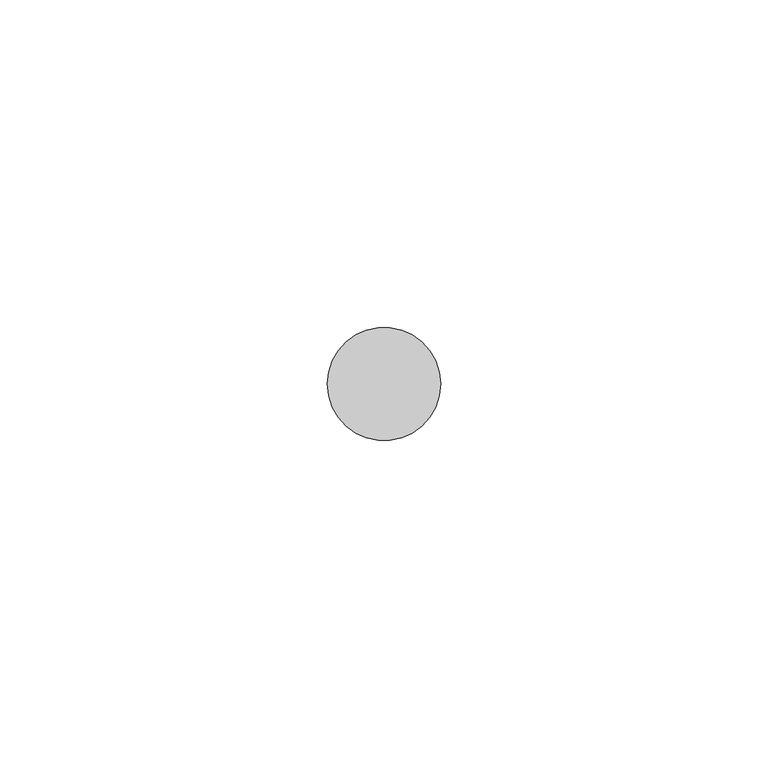
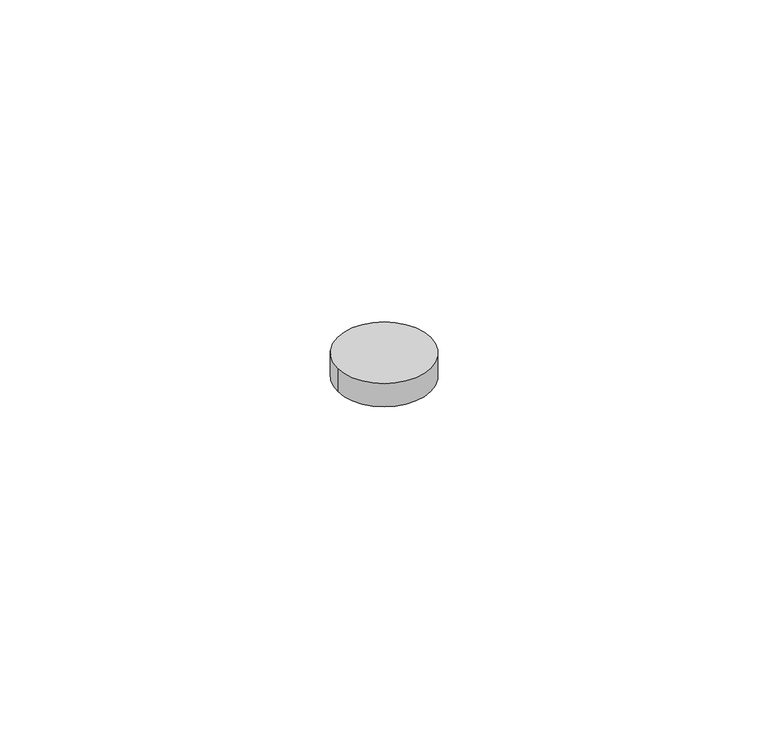
"""IFC4 building model written with IfcOpenShell, lengths in millimetres: proxy geometry, Hinge Pin Keeper17 : Hinge Pin Keeper."""

import ifcopenshell
import ifcopenshell.guid

model = None  # the IFC model being written
_history = None  # IfcOwnerHistory: only IFC2X3 demands one
_inside = {}  # id of a spatial element -> (the spatial element, [elements in it])
_under = {}  # id of a project, library or spatial element -> (it, [spatial elements below it])
_declared = {}  # id of a project -> (the project, [libraries it declares])
_typed = {}  # id of a type object -> (the type object, [elements of that type])
_made_of = {}  # id of a material, layer set ... -> (it, [elements and type objects made of it])


def new_model(schema):
    """Start an empty IFC model of exactly this schema.

    Asked for "IFC4X3", IfcOpenShell would pick the latest addendum, in which some entities
    have other attributes; the version numbers below select the first issue.
    IFC2X3 requires an IfcOwnerHistory on every rooted entity: one is made here for all.
    """
    global model, _history
    if schema == "IFC4X3":
        model = ifcopenshell.file(schema_version=(4, 3, 0, 0))
    else:
        model = ifcopenshell.file(schema=schema)
    _inside.clear()
    _under.clear()
    _declared.clear()
    _typed.clear()
    _made_of.clear()
    _history = None
    if model.schema == "IFC2X3":
        org = make("IfcOrganization", Name="unknown")
        user = make(
            "IfcPersonAndOrganization",
            ThePerson=make("IfcPerson", FamilyName="unknown"),
            TheOrganization=org,
        )
        app = make(
            "IfcApplication",
            ApplicationDeveloper=org,
            Version="unknown",
            ApplicationFullName="unknown",
            ApplicationIdentifier="unknown",
        )
        _history = make(
            "IfcOwnerHistory",
            OwningUser=user,
            OwningApplication=app,
            ChangeAction="ADDED",
            CreationDate=0,
        )
    return model


def make(cls, **values):
    """One entity of the class cls with the attributes given. An attribute that is None is left unset."""
    return model.create_entity(
        cls, **{name: value for name, value in values.items() if value is not None}
    )


def rooted(cls, **values):
    """An entity with a GlobalId (a new one), such as an element, a storey or a relation."""
    return make(cls, GlobalId=ifcopenshell.guid.new(), OwnerHistory=_history, **values)


def si_unit(unit_type, name, prefix=None):
    """IfcSIUnit, for example si_unit("LENGTHUNIT", "METRE", prefix="MILLI")."""
    return make("IfcSIUnit", UnitType=unit_type, Prefix=prefix, Name=name)


def assignment(units):
    """IfcUnitAssignment: the units of a project."""
    return None if units is None else make("IfcUnitAssignment", Units=units)


def point(xyz):
    """IfcCartesianPoint."""
    return None if xyz is None else make("IfcCartesianPoint", Coordinates=xyz)


def direction(xyz):
    """IfcDirection."""
    return None if xyz is None else make("IfcDirection", DirectionRatios=xyz)


def frame(location, z_axis=None, x_axis=None):
    """IfcAxis2Placement3D, a coordinate frame: its origin and axes. An axis left out is left unset."""
    return make(
        "IfcAxis2Placement3D",
        Location=point(location),
        Axis=direction(z_axis),
        RefDirection=direction(x_axis),
    )


def frame_2d(location, x_axis=None):
    """IfcAxis2Placement2D, a coordinate frame in the plane: its origin and x axis."""
    return make(
        "IfcAxis2Placement2D", Location=point(location), RefDirection=direction(x_axis)
    )


def origin():
    """The frame at (0, 0, 0) with its axes left unset."""
    return frame((0.0, 0.0, 0.0))


def place(relative_to, where):
    """IfcLocalPlacement: puts the frame where relative to a parent placement (None: the world)."""
    return make(
        "IfcLocalPlacement", PlacementRelTo=relative_to, RelativePlacement=where
    )


def context(
    kind, dimensions, precision=None, world=None, true_north=None, identifier=None
):
    """IfcGeometricRepresentationContext, for example the 3D "Model" context."""
    return make(
        "IfcGeometricRepresentationContext",
        ContextIdentifier=identifier,
        ContextType=kind,
        CoordinateSpaceDimension=dimensions,
        Precision=precision,
        WorldCoordinateSystem=world,
        TrueNorth=true_north,
    )


def project(units=None, contexts=None):
    """IfcProject with its units and contexts."""
    return rooted(
        "IfcProject",
        Name="project",
        RepresentationContexts=contexts,
        UnitsInContext=assignment(units),
    )


def spatial(cls, under=None, at=None, **own):
    """A site, building, storey or space (cls), placed at a placement, below another one or the project."""
    s = rooted(cls, ObjectPlacement=at, **own)
    if under is not None:
        _under.setdefault(under.id(), (under, []))[1].append(s)
    return s


def circle_curve(where, radius):
    """IfcCircle in the frame where."""
    return make("IfcCircle", Position=where, Radius=radius)


def trimmed(basis, trim1, trim2, sense, master):
    """IfcTrimmedCurve: the piece of a basis curve between two trims."""
    return make(
        "IfcTrimmedCurve",
        BasisCurve=basis,
        Trim1=trim1,
        Trim2=trim2,
        SenseAgreement=sense,
        MasterRepresentation=master,
    )


def segment(curve, same_sense, transition):
    """IfcCompositeCurveSegment."""
    return make(
        "IfcCompositeCurveSegment",
        Transition=transition,
        SameSense=same_sense,
        ParentCurve=curve,
    )


def composite_curve(segments, self_intersect=None):
    """IfcCompositeCurve: segments joined end to end."""
    return make("IfcCompositeCurve", Segments=segments, SelfIntersect=self_intersect)


def outline(outer, holes=None, kind="AREA"):
    """IfcArbitraryClosedProfileDef: a profile drawn as a closed curve; with holes, ...WithVoids."""
    if holes is None:
        return make("IfcArbitraryClosedProfileDef", ProfileType=kind, OuterCurve=outer)
    return make(
        "IfcArbitraryProfileDefWithVoids",
        ProfileType=kind,
        OuterCurve=outer,
        InnerCurves=holes,
    )


def extrude(swept, where, along, depth):
    """IfcExtrudedAreaSolid: the profile swept, set in the frame where, extruded along a direction by depth."""
    return make(
        "IfcExtrudedAreaSolid",
        SweptArea=swept,
        Position=where,
        ExtrudedDirection=direction(along),
        Depth=depth,
    )


def shape(context_of_items, identifier, shape_type, items):
    """IfcShapeRepresentation: the items that make up one representation, for example the "Body"."""
    return make(
        "IfcShapeRepresentation",
        ContextOfItems=context_of_items,
        RepresentationIdentifier=identifier,
        RepresentationType=shape_type,
        Items=items,
    )


def source(mapping_origin, context_of_items, identifier, shape_type, items):
    """IfcRepresentationMap: a shape defined once, which mapped items show again and again."""
    return make(
        "IfcRepresentationMap",
        MappingOrigin=mapping_origin,
        MappedRepresentation=shape(context_of_items, identifier, shape_type, items),
    )


def transform(
    local_origin,
    x_axis=None,
    y_axis=None,
    z_axis=None,
    scale=None,
    scale2=None,
    scale3=None,
    uniform=True,
):
    """IfcCartesianTransformationOperator3D, or its non-uniform kind. x_axis, y_axis, z_axis: its Axis1, 2, 3."""
    if uniform:
        return make(
            "IfcCartesianTransformationOperator3D",
            Axis1=direction(x_axis),
            Axis2=direction(y_axis),
            LocalOrigin=point(local_origin),
            Scale=scale,
            Axis3=direction(z_axis),
        )
    return make(
        "IfcCartesianTransformationOperator3DnonUniform",
        Axis1=direction(x_axis),
        Axis2=direction(y_axis),
        LocalOrigin=point(local_origin),
        Scale=scale,
        Axis3=direction(z_axis),
        Scale2=scale2,
        Scale3=scale3,
    )


def mapped(mapping_source, mapping_target):
    """IfcMappedItem: shows the shape of a source again, moved by a transform."""
    return make(
        "IfcMappedItem", MappingSource=mapping_source, MappingTarget=mapping_target
    )


def made_of(thing, what):
    """Note that an element or type object is made of a material, layer set ...; save() writes the relation."""
    if what is not None:
        _made_of.setdefault(what.id(), (what, []))[1].append(thing)
    return thing


def element(
    cls,
    number,
    at=None,
    inside=None,
    cuts=None,
    type_object=None,
    material=None,
    context=None,
    identifier="Body",
    shape_type=None,
    held_by="IfcProductDefinitionShape",
    body=None,
    shapes=None,
    **own,
):
    """One element of the class cls, such as IfcWall. Its Tag is "e" and its number.

    at: its placement. inside: the storey or other place that contains it. cuts: it is an
    opening in that element (IfcRelVoidsElement). A single representation is given by context,
    identifier, shape_type and body (its items); several are given by shapes. held_by: the class
    of the entity that holds the representations. save() writes the other relations.
    """
    e = rooted(cls, Tag="e%d" % number, ObjectPlacement=at, **own)
    if body is not None:
        shapes = [shape(context, identifier, shape_type, body)]
    if shapes is not None:
        e.Representation = make(held_by, Representations=shapes)
    if inside is not None:
        _inside.setdefault(inside.id(), (inside, []))[1].append(e)
    if cuts is not None:
        rooted(
            "IfcRelVoidsElement", RelatingBuildingElement=cuts, RelatedOpeningElement=e
        )
    if type_object is not None:
        _typed.setdefault(type_object.id(), (type_object, []))[1].append(e)
    return made_of(e, material)


def aggregate(whole, parts):
    """IfcRelAggregates: a whole, such as a stair, and the parts it consists of."""
    return rooted("IfcRelAggregates", RelatingObject=whole, RelatedObjects=parts)


def save(model, path):
    """Write the relations noted so far, then the file.

    IfcRelAggregates (storeys below a building ...), IfcRelContainedInSpatialStructure (elements
    in a storey), IfcRelDefinesByType, IfcRelAssociatesMaterial and IfcRelDeclares: one each for
    every whole, place, type object, material and project.
    """
    for whole, parts in _under.values():
        aggregate(whole, parts)
    for where, things in _inside.values():
        rooted(
            "IfcRelContainedInSpatialStructure",
            RelatedElements=things,
            RelatingStructure=where,
        )
    for kind, things in _typed.values():
        rooted("IfcRelDefinesByType", RelatedObjects=things, RelatingType=kind)
    for what, things in _made_of.values():
        rooted("IfcRelAssociatesMaterial", RelatedObjects=things, RelatingMaterial=what)
    for by, libraries in _declared.values():
        rooted("IfcRelDeclares", RelatingContext=by, RelatedDefinitions=libraries)
    model.write(path)


def generic_models_87e8abe8(model_context):
    return source(origin(), model_context, "Body", "SweptSolid", [
        extrude(outline(composite_curve([segment(trimmed(circle_curve(frame_2d((587319.1320739, -533984.6777841)), 8.6534625), [point((587310.4786114, -533984.6777841))], [point((587327.7855364, -533984.6777841))], False, "CARTESIAN"), True, "CONTINUOUS"), segment(trimmed(circle_curve(frame_2d((587319.1320739, -533984.6777841)), 8.6534625), [point((587327.7855364, -533984.6777841))], [point((587310.4786114, -533984.6777841))], False, "CARTESIAN"), True, "CONTINUOUS")], self_intersect=False)), frame((0.0, 0.0, 1271.7859375), z_axis=(0.0, 0.0, 1.0), x_axis=(1.0, 0.0, 0.0)), (0.0, 0.0, 1.0), 4.5640625),
    ])


if __name__ == "__main__":
    model = new_model("IFC4")
    model_context = context("Model", 3, world=origin())
    ifc_project = project(units=[si_unit("LENGTHUNIT", "METRE", prefix="MILLI")], contexts=[model_context])
    site = spatial("IfcSite", under=ifc_project)
    building = spatial("IfcBuilding", under=site)
    placement = place(None, origin())
    generic_models_shape = generic_models_87e8abe8(model_context)
    element("IfcBuildingElementProxy", 1, Name="Hinge Pin Keeper17 : Hinge Pin Keeper", ObjectType="Hinge Pin Keeper17 : Hinge Pin Keeper", at=placement, inside=building, context=model_context, shape_type="MappedRepresentation", body=[
        mapped(generic_models_shape, transform((0.0, 0.0, 0.0), x_axis=(1.0, 0.0, 0.0), y_axis=(0.0, 1.0, 0.0), z_axis=(0.0, 0.0, 1.0))),
    ])
    save(model, "model.ifc")

# Revit data of these elements
# Element 1 (IfcBuildingElementProxy, "Hinge Pin Keeper17 : Hinge Pin Keeper")
#   Materials on its faces: "6\"X6\" WELD-ON STL BUTT HINGE"
# Materials
#   "6\"X6\" WELD-ON STL BUTT HINGE": class "Metal", colour RGB 189 187 185, transparency 0, Description = "Carbon steel", Cost = 0
